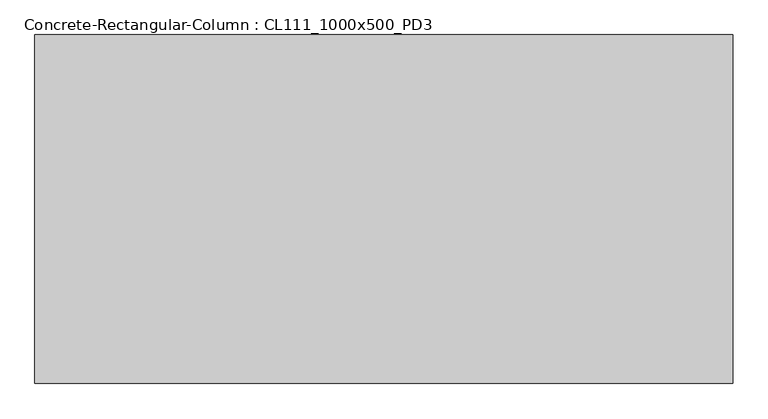
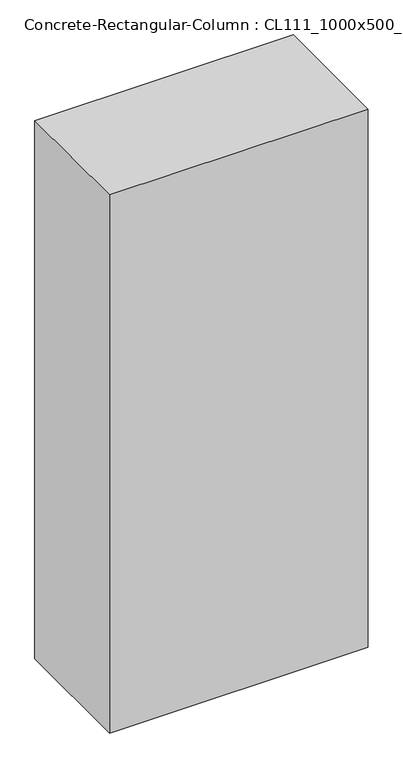
"""IFC4 building model written with IfcOpenShell, lengths in millimetres: column geometry, Concrete-Rectangular-Column : CL111_1000x500_PD3."""

from ifc_helpers import new_model, si_unit, frame, origin, place, context, project, spatial, polyline, outline, extrude, source, transform, mapped, element, save


def concrete_rectangular_column_cl111_1000x500_pd3_b8057e20(model_context):
    return source(origin(), model_context, "Body", "SweptSolid", [
        extrude(outline(polyline([(500.0, 250.0), (500.0, -250.0), (-500.0, -250.0), (-500.0, 250.0), (500.0, 250.0)])), frame((0.0, 0.0, -2100.0), z_axis=(0.0, 0.0, 1.0), x_axis=(1.0, 0.0, 0.0)), (0.0, 0.0, 1.0), 2200.0),
    ])


if __name__ == "__main__":
    model = new_model("IFC4")
    model_context = context("Model", 3, world=origin())
    ifc_project = project(units=[si_unit("LENGTHUNIT", "METRE", prefix="MILLI")], contexts=[model_context])
    site = spatial("IfcSite", under=ifc_project)
    building = spatial("IfcBuilding", under=site)
    placement = place(None, origin())
    concrete_rectangular_column_cl111_1000x500_pd3_shape = concrete_rectangular_column_cl111_1000x500_pd3_b8057e20(model_context)
    element("IfcColumn", 1, ObjectType="Concrete-Rectangular-Column : CL111_1000x500_PD3", at=placement, inside=building, context=model_context, shape_type="MappedRepresentation", body=[
        mapped(concrete_rectangular_column_cl111_1000x500_pd3_shape, transform((0.0, 0.0, 0.0), x_axis=(1.0, 0.0, 0.0), y_axis=(0.0, 1.0, 0.0), z_axis=(0.0, 0.0, 1.0))),
    ])
    save(model, "model.ifc")

# Revit data of these elements
# Type "Concrete-Rectangular-Column : CL111_1000x500_PD3"
#   Description = "UG 철골 기둥용 Pedestal"
#   b = 1000 mm
#   h = 500 mm
#   Width = 1000 mm
#   Length = 500 mm
#   hec_material3 [instance default] = none
#   hec_material2 [instance default] = A03AE056-00001_Bitumen/Bituminous/Asphalt Coating
#   hec_material1 [instance default] = A03AC035-00001_Form Work (3 times in use)_Flat
#   Structural Material [instance default] = A03AC032-00007_Structural Concrete_Type1_25MPa-30Mpa
# Element 1 (IfcColumn, "Concrete-Rectangular-Column : CL111_1000x500_PD3")
#   hec_material2 = none
#   hec_material1 = none
#   Structural Material = 콘크리트 - 현장타설 콘크리트
#   Materials on its faces: "콘크리트 - 현장타설 콘크리트"
# Materials
#   "A03AE056-00001_Bitumen/Bituminous/Asphalt Coating": class "Generic", colour RGB 17 17 17, transparency 0, Description = "Damp-proofing", W00) Work Master Code = "A03AE056-00001", W01) Work Master_Lv1 = "Concrete Work", W02) Work Master_Lv2 = "Concrete Protective Coating (U/G)", W03) Work Master_Spec.1 = "Bitumen/Bituminous/Asphalt Coating", Cost = 0
#   "A03AC035-00001_Form Work (3 times in use)_Flat": class "Wood", colour RGB 149 120 74, transparency 0, Description = "Plywood", W00) Work Master Code = "A03AC035-00001", W01) Work Master_Lv1 = "Concrete Work", W02) Work Master_Lv2 = "Substructure Work", W03) Work Master_Spec.1 = "Form Work (3 times in use)", W04) Work Master_Spec.2 = "Flat Form", W05) Work Master_Spec.3 = "Dressed Lumber, Plywood or Steel Form(Wood Planks are not Allowed) incl. Chamfer", Cost = 0
#   "A03AC032-00007_Structural Concrete_Type1_25MPa-30Mpa": class "Concrete", colour RGB 176 176 176, transparency 0, Keynote = "09910.A1", Description = "Reinf. Conc.", W00) Work Master Code = "A03AC032-00007", W01) Work Master_Lv1 = "Concrete Work", W02) Work Master_Lv2 = "Substructure Work", W03) Work Master_Spec.1 = "Structural Concrete", W04) Work Master_Spec.2 = "Cement Type-1", W05) Work Master_Spec.3 = "25MPa < F'c (Cylinder Strength) ≤ 30MPa", Cost = 0
#   "콘크리트 - 현장타설 콘크리트": class "콘크리트", colour RGB 192 192 192, transparency 0
